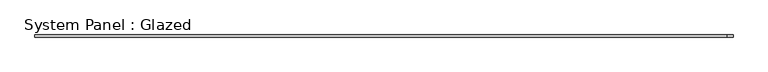
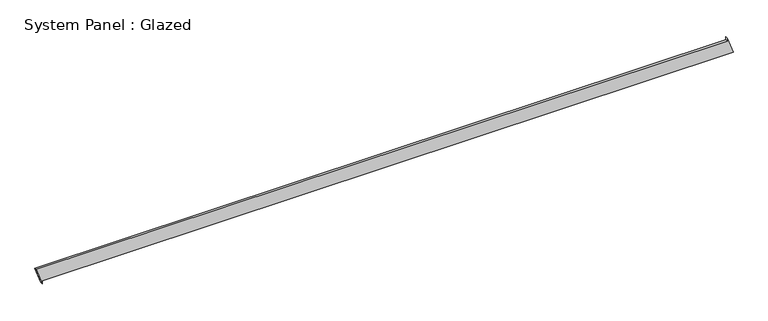
"""IFC4 building model written with IfcOpenShell, lengths in millimetres: plate geometry, System Panel : Glazed."""

from ifc_helpers import new_model, si_unit, frame, origin, place, context, project, spatial, polyline, outline, extrude, source, transform, mapped, element, save


def system_panel_glazed_6789d7e7(model_context):
    return source(origin(), model_context, "Body", "SweptSolid", [
        extrude(outline(polyline([(0.0, -3958.2435347), (35.3553391, -3958.2435347), (35.3553391, 4027.3171494), (234.739942, 3958.6129922), (199.3846029, 3958.613671), (199.2312647, -4027.3171494), (0.0, -3958.2435347)])), frame((0.0, -49.5, 0.0), z_axis=(0.0, 1.0, 0.0), x_axis=(0.0, 0.0, 1.0)), (0.0, 0.0, 1.0), 25.0),
    ])


if __name__ == "__main__":
    model = new_model("IFC4")
    model_context = context("Model", 3, world=origin())
    ifc_project = project(units=[si_unit("LENGTHUNIT", "METRE", prefix="MILLI")], contexts=[model_context])
    site = spatial("IfcSite", under=ifc_project)
    building = spatial("IfcBuilding", under=site)
    placement = place(None, origin())
    system_panel_glazed_shape = system_panel_glazed_6789d7e7(model_context)
    element("IfcPlate", 1, ObjectType="System Panel : Glazed", at=placement, inside=building, context=model_context, shape_type="MappedRepresentation", body=[
        mapped(system_panel_glazed_shape, transform((0.0, 0.0, 0.0), x_axis=(1.0, 0.0, 0.0), y_axis=(0.0, 1.0, 0.0), z_axis=(0.0, 0.0, 1.0))),
    ])
    save(model, "model.ifc")

# Revit data of these elements
# Element 1 (IfcPlate, "System Panel : Glazed")
#   Materials on its faces: "Glass"
# Materials
#   "Glass": class "Glass", colour RGB 218 227 224, transparency 0.85, Description = "Soda Lime Glass", Cost = 0
